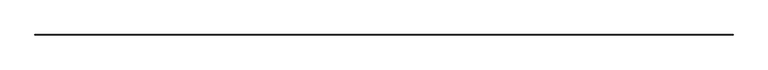
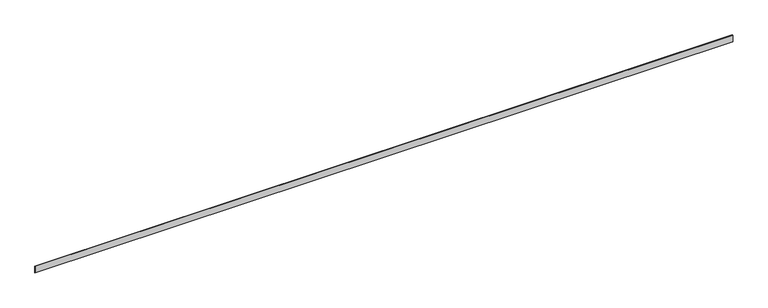
"""IFC4 building model written with IfcOpenShell, lengths in millimetres: proxy geometry, Generic Models 7:Generic Models 1:337419:Generic Models 1:337419 : Generic Models 7:Generic Models 1:337419:21 : Generic Models 7:Generic Models 1:337419:Generic Models 1:337419 : Generic Models 7:Generic Models 1:337419:301336."""

from ifc_helpers import new_model, si_unit, frame, origin, place, context, project, spatial, polyline, outline, extrude, source, transform, mapped, element, save


def generic_models_c842a5f0(model_context):
    return source(origin(), model_context, "Body", "SweptSolid", [
        extrude(outline(polyline([(596182.8367242, -568186.6413841), (596182.8367242, -568189.8163841), (591306.0367242, -568189.8163841), (591306.0367242, -568186.6413841), (596182.8367242, -568186.6413841)])), frame((0.0, 0.0, 4851.453012), z_axis=(0.0, 0.0, 1.0), x_axis=(1.0, 0.0, 0.0)), (0.0, 0.0, 1.0), 48.1210938),
    ])


if __name__ == "__main__":
    model = new_model("IFC4")
    model_context = context("Model", 3, world=origin())
    ifc_project = project(units=[si_unit("LENGTHUNIT", "METRE", prefix="MILLI")], contexts=[model_context])
    site = spatial("IfcSite", under=ifc_project)
    building = spatial("IfcBuilding", under=site)
    placement = place(None, origin())
    generic_models_shape = generic_models_c842a5f0(model_context)
    element("IfcBuildingElementProxy", 1, Name="Generic Models 7:Generic Models 1:337419:Generic Models 1:337419 : Generic Models 7:Generic Models 1:337419:21 : Generic Models 7:Generic Models 1:337419:Generic Models 1:337419 : Generic Models 7:Generic Models 1:337419:301336", ObjectType="Generic Models 7:Generic Models 1:337419:Generic Models 1:337419 : Generic Models 7:Generic Models 1:337419:21 : Generic Models 7:Generic Models 1:337419:Generic Models 1:337419 : Generic Models 7:Generic Models 1:337419:301336", at=placement, inside=building, context=model_context, shape_type="MappedRepresentation", body=[
        mapped(generic_models_shape, transform((0.0, 0.0, 0.0), x_axis=(1.0, 0.0, 0.0), y_axis=(0.0, 1.0, 0.0), z_axis=(0.0, 0.0, 1.0))),
    ])
    save(model, "model.ifc")

# Revit data of these elements
# Type "Generic Models 7:Generic Models 1:337419:Generic Models 1:337419 : Generic Models 7:Generic Models 1:337419:21 : Generic Models 7:Generic Models 1:337419:Generic Models 1:337419 : Generic Models 7:Generic Models 1:337419:301336"
#   NameOverride = "Generic Models 7:Generic Models 1:337419:Generic Models 1:337419 : Generic Models 7:Generic Models 1:337419:301336"
#   ObjectTypeOverride = "Generic Models 1:337419 : Generic Models 7:Generic Models 1:337419"
#   Reference = "Generic Models 1"
#   Tag = "301336"
# Element 1 (IfcBuildingElementProxy, "Generic Models 7:Generic Models 1:337419:Generic Models 1:337419 : Generic Models 7:Generic Models 1:337419:21 : Generic Models 7:Generic Models 1:337419:Generic Models 1:337419 : Generic Models 7:Generic Models 1:337419:301336")
#   Materials on its faces: "COMPRESSIBE THERMAL GASKET SANDWICHED BETWEEN METAL COMPONENTS"
# Materials
#   "COMPRESSIBE THERMAL GASKET SANDWICHED BETWEEN METAL COMPONENTS": class "Unassigned", colour RGB 58 208 21, transparency 0, Cost = 0
